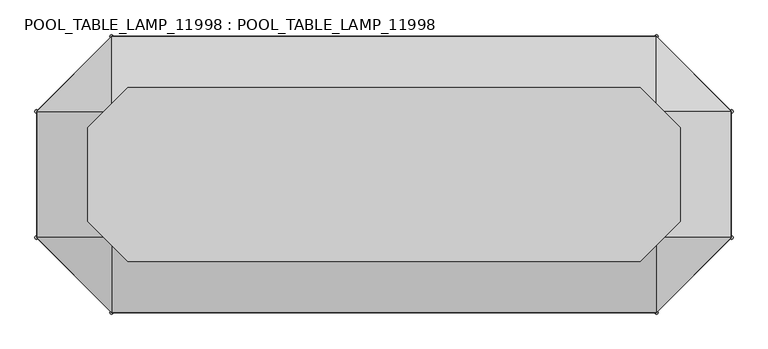
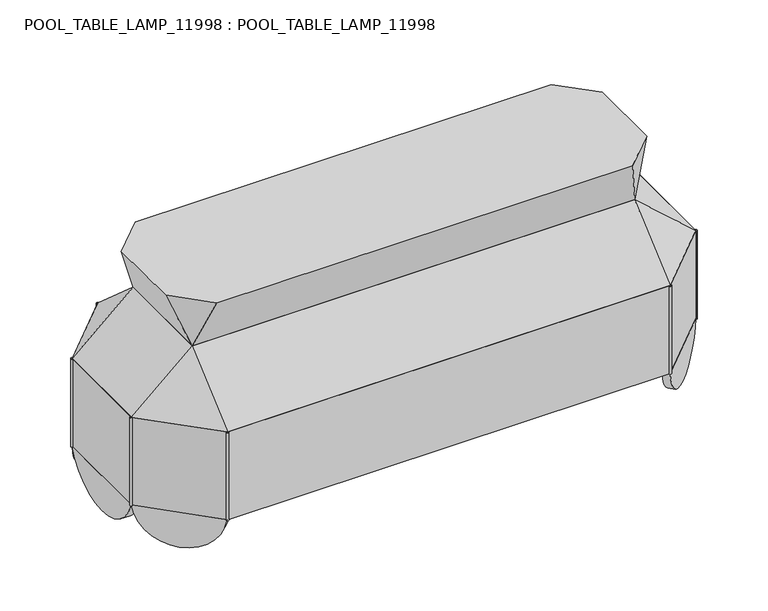
"""IFC4 building model written with IfcOpenShell, lengths in millimetres: proxy geometry, POOL_TABLE_LAMP_11998 : POOL_TABLE_LAMP_11998."""

from ifc_helpers import new_model, si_unit, point, frame, frame_2d, origin, place, context, project, spatial, polyline, circle_curve, trimmed, segment, composite_curve, outline, extrude, faceted_brep, source, transform, mapped, element, save


def pool_table_lamp_11998_pool_table_lamp_11998_d06ee5fc(model_context):
    return source(origin(), model_context, "Body", "SolidModel", [
        extrude(outline(composite_curve([segment(trimmed(circle_curve(frame_2d((246.5034627, 1717.728225)), 130.228225), [point((369.9998934, 1676.4))], [point((123.007032, 1676.4))], False, "CARTESIAN"), True, "CONTINUOUS"), segment(polyline([(123.007032, 1676.4), (369.9998934, 1676.4)]), True, "CONTINUOUS")], self_intersect=False)), frame((-1365.4872204, 0.0, 0.0), z_axis=(1.0, 0.0, 0.0), x_axis=(0.0, 1.0, 0.0)), (0.0, 0.0, 1.0), 24.3292268),
        extrude(outline(composite_curve([segment(polyline([(1676.4, -151.8960871), (1676.4, -685.2960871)]), True, "CONTINUOUS"), segment(trimmed(circle_curve(frame_2d((2032.0, -418.5960871)), 444.5), [point((1676.4, -685.2960871))], [point((1676.4, -151.8960871))], False, "CARTESIAN"), True, "CONTINUOUS")], self_intersect=False)), frame((0.0, 493.0069254, 0.0), z_axis=(0.0, 1.0, 0.0), x_axis=(0.0, 0.0, 1.0)), (0.0, 0.0, 1.0), 24.3292268),
        extrude(outline(composite_curve([segment(trimmed(circle_curve(frame_2d((246.5034627, 1717.728225)), 130.228225), [point((369.9998934, 1676.4))], [point((123.007032, 1676.4))], False, "CARTESIAN"), True, "CONTINUOUS"), segment(polyline([(123.007032, 1676.4), (369.9998934, 1676.4)]), True, "CONTINUOUS")], self_intersect=False)), frame((-29.4341807, 0.0, 0.0), z_axis=(1.0, 0.0, 0.0), x_axis=(0.0, 1.0, 0.0)), (0.0, 0.0, 1.0), 24.3292268),
        extrude(outline(polyline([(-151.8960871, 493.0069254), (-1218.6960871, 493.0069254), (-1218.6960871, 517.3361522), (-151.8960871, 517.3361522), (-151.8960871, 493.0069254)])), frame((0.0, 0.0, 1676.4), z_axis=(0.0, 0.0, 1.0), x_axis=(1.0, 0.0, 0.0)), (0.0, 0.0, 1.0), 224.1601186),
        extrude(outline(polyline([(-1341.1579936, 123.007032), (-1365.4872204, 123.007032), (-1365.4872204, 369.9998934), (-1341.1579936, 369.9998934), (-1341.1579936, 123.007032)])), frame((0.0, 0.0, 1676.4), z_axis=(0.0, 0.0, 1.0), x_axis=(1.0, 0.0, 0.0)), (0.0, 0.0, 1.0), 224.1601186),
        extrude(outline(polyline([(-29.4341807, 123.007032), (-29.4341807, 369.9998934), (-5.1049539, 369.9998934), (-5.1049539, 123.007032), (-29.4341807, 123.007032)])), frame((0.0, 0.0, 1676.4), z_axis=(0.0, 0.0, 1.0), x_axis=(1.0, 0.0, 0.0)), (0.0, 0.0, 1.0), 224.1601186),
        extrude(outline(polyline([(-151.8960871, 0.0), (-151.8960871, -24.3292268), (-1218.6960871, -24.3292268), (-1218.6960871, 0.0), (-151.8960871, 0.0)])), frame((0.0, 0.0, 1676.4), z_axis=(0.0, 0.0, 1.0), x_axis=(1.0, 0.0, 0.0)), (0.0, 0.0, 1.0), 224.1601186),
        extrude(outline(composite_curve([segment(polyline([(-155.0710871, -24.0098052), (-148.7210871, -24.0098052)]), True, "CONTINUOUS"), segment(trimmed(circle_curve(frame_2d((-151.8960871, -24.0098052)), 3.175), [point((-148.7210871, -24.0098052))], [point((-155.0710871, -24.0098052))], False, "CARTESIAN"), True, "CONTINUOUS")], self_intersect=False)), frame((0.0, 0.0, 1676.4), z_axis=(0.0, 0.0, 1.0), x_axis=(1.0, 0.0, 0.0)), (0.0, 0.0, 1.0), 224.1601186),
        extrude(outline(composite_curve([segment(trimmed(circle_curve(frame_2d((-1218.6960871, -24.0098052)), 3.175), [point((-1215.5210871, -24.0098052))], [point((-1221.8710871, -24.0098052))], False, "CARTESIAN"), True, "CONTINUOUS"), segment(polyline([(-1221.8710871, -24.0098052), (-1215.5210871, -24.0098052)]), True, "CONTINUOUS")], self_intersect=False)), frame((0.0, 0.0, 1676.4), z_axis=(0.0, 0.0, 1.0), x_axis=(1.0, 0.0, 0.0)), (0.0, 0.0, 1.0), 224.1601186),
        extrude(outline(composite_curve([segment(polyline([(-1215.5210871, 517.0167306), (-1221.8710871, 517.0167306)]), True, "CONTINUOUS"), segment(trimmed(circle_curve(frame_2d((-1218.6960871, 517.0167306)), 3.175), [point((-1221.8710871, 517.0167306))], [point((-1215.5210871, 517.0167306))], False, "CARTESIAN"), True, "CONTINUOUS")], self_intersect=False)), frame((0.0, 0.0, 1676.4), z_axis=(0.0, 0.0, 1.0), x_axis=(1.0, 0.0, 0.0)), (0.0, 0.0, 1.0), 224.1601186),
        extrude(outline(composite_curve([segment(trimmed(circle_curve(frame_2d((-151.8960871, 517.0167306)), 3.175), [point((-155.0710871, 517.0167306))], [point((-148.7210871, 517.0167306))], False, "CARTESIAN"), True, "CONTINUOUS"), segment(polyline([(-148.7210871, 517.0167306), (-155.0710871, 517.0167306)]), True, "CONTINUOUS")], self_intersect=False)), frame((0.0, 0.0, 1676.4), z_axis=(0.0, 0.0, 1.0), x_axis=(1.0, 0.0, 0.0)), (0.0, 0.0, 1.0), 224.1601186),
        extrude(outline(composite_curve([segment(polyline([(-5.1049539, 119.6063281), (-5.1049539, 125.9563281)]), True, "CONTINUOUS"), segment(trimmed(circle_curve(frame_2d((-5.1049539, 122.7813281)), 3.175), [point((-5.1049539, 125.9563281))], [point((-5.1049539, 119.6063281))], False, "CARTESIAN"), True, "CONTINUOUS")], self_intersect=False)), frame((0.0, 0.0, 1676.4), z_axis=(0.0, 0.0, 1.0), x_axis=(1.0, 0.0, 0.0)), (0.0, 0.0, 1.0), 224.1601186),
        extrude(outline(composite_curve([segment(trimmed(circle_curve(frame_2d((-5.1049539, 370.2255973)), 3.175), [point((-5.1049539, 373.4005973))], [point((-5.1049539, 367.0505973))], False, "CARTESIAN"), True, "CONTINUOUS"), segment(polyline([(-5.1049539, 367.0505973), (-5.1049539, 373.4005973)]), True, "CONTINUOUS")], self_intersect=False)), frame((0.0, 0.0, 1676.4), z_axis=(0.0, 0.0, 1.0), x_axis=(1.0, 0.0, 0.0)), (0.0, 0.0, 1.0), 224.1601186),
        extrude(outline(composite_curve([segment(polyline([(-1365.4872204, 373.4005973), (-1365.4872204, 367.0505973)]), True, "CONTINUOUS"), segment(trimmed(circle_curve(frame_2d((-1365.4872204, 370.2255973)), 3.175), [point((-1365.4872204, 367.0505973))], [point((-1365.4872204, 373.4005973))], False, "CARTESIAN"), True, "CONTINUOUS")], self_intersect=False)), frame((0.0, 0.0, 1676.4), z_axis=(0.0, 0.0, 1.0), x_axis=(1.0, 0.0, 0.0)), (0.0, 0.0, 1.0), 224.1601186),
        extrude(outline(composite_curve([segment(trimmed(circle_curve(frame_2d((-1365.4872204, 122.7813281)), 3.175), [point((-1365.4872204, 119.6063281))], [point((-1365.4872204, 125.9563281))], False, "CARTESIAN"), True, "CONTINUOUS"), segment(polyline([(-1365.4872204, 125.9563281), (-1365.4872204, 119.6063281)]), True, "CONTINUOUS")], self_intersect=False)), frame((0.0, 0.0, 1676.4), z_axis=(0.0, 0.0, 1.0), x_axis=(1.0, 0.0, 0.0)), (0.0, 0.0, 1.0), 224.1601186),
        extrude(outline(composite_curve([segment(polyline([(-207.9132051, 0.0), (0.0, 0.0)]), True, "CONTINUOUS"), segment(trimmed(circle_curve(frame_2d((-103.9566025, 16.3316378)), 105.2316378), [point((0.0, 0.0))], [point((-207.9132051, 0.0))], False, "CARTESIAN"), True, "CONTINUOUS")], self_intersect=False)), frame((-1365.7129243, 123.007032, 1676.4), z_axis=(0.7071067811865518, 0.7071067811865434, 0.0), x_axis=(-0.7071067811865434, 0.7071067811865518, 0.0)), (0.0, 0.0, 1.0), 17.362958),
        extrude(outline(composite_curve([segment(trimmed(circle_curve(frame_2d((0.0, -105.2316378)), 105.2316378), [point((-85.0566304, -167.1918446))], [point((61.9602067, -20.1750074))], False, "CARTESIAN"), True, "CONTINUOUS"), segment(polyline([(61.9602067, -20.1750074), (-85.0566304, -167.1918446)]), True, "CONTINUOUS")], self_intersect=False)), frame((-25.7718496, 102.1144323, 1618.3216331), z_axis=(-0.7071067811865426, 0.7071067811865525, 0.0), x_axis=(0.5000000000000033, 0.4999999999999975, 0.7071067811865469)), (0.0, 0.0, 1.0), 17.362958),
        extrude(outline(composite_curve([segment(polyline([(85.0566304, -167.1918446), (-61.9602067, -20.1750074)]), True, "CONTINUOUS"), segment(trimmed(circle_curve(frame_2d((0.0, -105.2316378)), 105.2316378), [point((-61.9602067, -20.1750074))], [point((85.0566304, -167.1918446))], False, "CARTESIAN"), True, "CONTINUOUS")], self_intersect=False)), frame((-1332.5428593, 378.6150278, 1618.3216331), z_axis=(-0.7071067811865472, 0.7071067811865479, 0.0), x_axis=(0.5000000000000001, 0.5000000000000009, -0.707106781186547)), (0.0, 0.0, 1.0), 17.362958),
        extrude(outline(composite_curve([segment(trimmed(circle_curve(frame_2d((103.9566025, 16.3316378)), 105.2316378), [point((207.9132051, 0.0))], [point((0.0, 0.0))], False, "CARTESIAN"), True, "CONTINUOUS"), segment(polyline([(0.0, 0.0), (207.9132051, 0.0)]), True, "CONTINUOUS")], self_intersect=False)), frame((-17.1567153, 357.7224281, 1676.4), z_axis=(0.7071067811865472, 0.7071067811865479, 0.0), x_axis=(-0.7071067811865479, 0.7071067811865472, 0.0)), (0.0, 0.0, 1.0), 17.362958),
        faceted_brep([(-1218.3766655, 123.007032, 2030.7043208), (-152.2155087, 123.007032, 2030.7043208), (-152.2155087, 369.9998934, 2030.7043208), (-1218.3766655, 369.9998934, 2030.7043208), (-177.484535, 148.453943, 2030.7043208), (-177.6630544, 148.2754236, 2030.7043208), (-1192.9291198, 148.2754236, 2030.7043208), (-1193.1076392, 148.453943, 2030.7043208), (-1193.1076392, 344.5529824, 2030.7043208), (-1192.9291198, 344.7315018, 2030.7043208), (-177.6630544, 344.7315018, 2030.7043208), (-177.484535, 344.5529824, 2030.7043208), (-1365.4872204, 122.7813281, 1900.5601186), (-1365.4872204, 370.2255973, 1900.5601186), (-1218.3766655, 517.3361522, 1900.5601186), (-152.2155087, 517.3361522, 1900.5601186), (-5.1049539, 370.2255973, 1900.5601186), (-5.1049539, 122.7813281, 1900.5601186), (-152.2155087, -24.3292268, 1900.5601186), (-1218.3766655, -24.3292268, 1900.5601186), (-152.4412126, 0.0, 1900.5601186), (-29.4341807, 123.007032, 1900.5601186), (-29.4341807, 369.9998934, 1900.5601186), (-152.4412126, 493.0069254, 1900.5601186), (-1218.1509616, 493.0069254, 1900.5601186), (-1341.1579936, 369.9998934, 1900.5601186), (-1341.1579936, 123.007032, 1900.5601186), (-1218.1509616, 0.0, 1900.5601186), (-177.6155087, 148.407032, 2030.2376392), (-177.6155087, 344.5998934, 2030.2376392), (-1192.9766655, 344.5998934, 2030.2376392), (-1192.9766655, 148.407032, 2030.2376392)], [[[0, 1, 2, 3], [4, 5, 6, 7, 8, 9, 10, 11]], [[12, 13, 14, 15, 16, 17, 18, 19], [20, 21, 22, 23, 24, 25, 26, 27]], [[12, 19, 0]], [[1, 0, 19, 18]], [[18, 17, 1]], [[2, 1, 17, 16]], [[16, 15, 2]], [[3, 2, 15, 14]], [[14, 13, 3]], [[0, 3, 13, 12]], [[4, 28, 5]], [[28, 4, 11, 29]], [[29, 11, 10]], [[29, 10, 9, 30]], [[30, 9, 8]], [[30, 8, 7, 31]], [[31, 7, 6]], [[5, 28, 31, 6]], [[20, 28, 21]], [[21, 28, 29, 22]], [[22, 29, 23]], [[23, 29, 30, 24]], [[24, 30, 25]], [[25, 30, 31, 26]], [[26, 31, 27]], [[28, 20, 27, 31]]]),
        extrude(outline(polyline([(-151.8960871, -24.0098052), (-151.8960871, 0.5451255), (-29.4341807, 123.007032), (-4.87925, 123.007032), (-151.8960871, -24.0098052)])), frame((0.0, 0.0, 1676.4), z_axis=(0.0, 0.0, 1.0), x_axis=(1.0, 0.0, 0.0)), (0.0, 0.0, 1.0), 224.1601186),
        extrude(outline(polyline([(-151.8960871, 517.0167306), (-4.87925, 369.9998934), (-29.4341807, 369.9998934), (-151.8960871, 492.4617999), (-151.8960871, 517.0167306)])), frame((0.0, 0.0, 1676.4), z_axis=(0.0, 0.0, 1.0), x_axis=(1.0, 0.0, 0.0)), (0.0, 0.0, 1.0), 224.1601186),
        extrude(outline(polyline([(-1218.6960871, 517.0167306), (-1218.6960871, 492.4617999), (-1341.1579936, 369.9998934), (-1365.7129243, 369.9998934), (-1218.6960871, 517.0167306)])), frame((0.0, 0.0, 1676.4), z_axis=(0.0, 0.0, 1.0), x_axis=(1.0, 0.0, 0.0)), (0.0, 0.0, 1.0), 224.1601186),
        extrude(outline(polyline([(-1218.6960871, -24.0098052), (-1365.7129243, 123.007032), (-1341.1579936, 123.007032), (-1218.6960871, 0.5451255), (-1218.6960871, -24.0098052)])), frame((0.0, 0.0, 1676.4), z_axis=(0.0, 0.0, 1.0), x_axis=(1.0, 0.0, 0.0)), (0.0, 0.0, 1.0), 224.1601186),
        faceted_brep([(-1186.5878882, 416.8069254, 2157.1484202), (-1264.9579936, 338.43682, 2157.1484202), (-1264.9579936, 154.5701054, 2157.1484202), (-1186.5878882, 76.2, 2157.1484202), (-184.0042861, 76.2, 2157.1484202), (-105.6341807, 154.5701054, 2157.1484202), (-105.6341807, 338.43682, 2157.1484202), (-184.0042861, 416.8069254, 2157.1484202), (-1218.3766655, 369.9998934, 2030.2376392), (-152.2155087, 369.9998934, 2030.2376392), (-152.2155087, 123.007032, 2030.2376392), (-1218.3766655, 123.007032, 2030.2376392)], [[[0, 1, 2, 3, 4, 5, 6, 7]], [[8, 9, 10, 11]], [[1, 0, 8]], [[8, 11, 2, 1]], [[3, 2, 11]], [[11, 10, 4, 3]], [[5, 4, 10]], [[10, 9, 6, 5]], [[7, 6, 9]], [[9, 8, 0, 7]]]),
    ])


if __name__ == "__main__":
    model = new_model("IFC4")
    model_context = context("Model", 3, world=origin())
    ifc_project = project(units=[si_unit("LENGTHUNIT", "METRE", prefix="MILLI")], contexts=[model_context])
    site = spatial("IfcSite", under=ifc_project)
    building = spatial("IfcBuilding", under=site)
    placement = place(None, origin())
    pool_table_lamp_11998_pool_table_lamp_11998_shape = pool_table_lamp_11998_pool_table_lamp_11998_d06ee5fc(model_context)
    element("IfcBuildingElementProxy", 1, Name="POOL_TABLE_LAMP_11998 : POOL_TABLE_LAMP_11998", ObjectType="POOL_TABLE_LAMP_11998 : POOL_TABLE_LAMP_11998", at=placement, inside=building, context=model_context, shape_type="MappedRepresentation", body=[
        mapped(pool_table_lamp_11998_pool_table_lamp_11998_shape, transform((0.0, 0.0, 0.0), x_axis=(1.0, 0.0, 0.0), y_axis=(0.0, 1.0, 0.0), z_axis=(0.0, 0.0, 1.0))),
    ])
    save(model, "model.ifc")

# Revit data of these elements
# Type "POOL_TABLE_LAMP_11998 : POOL_TABLE_LAMP_11998"
#   COBie.Type.CreatedBy = "design@eagle.com"
#   COBie.Type.CreatedOn = "2016-10-27T05:31:12"
#   COBie.Type.Name = "POOL_TABLE_LAMP_11998_POOL_TABLE_LAMP_11998"
#   COBie.Type.Category = "n/a"
#   COBie.Type.Description = "POOL_TABLE_LAMP_11998_POOL_TABLE_LAMP_11998"
#   COBie.Type.Manufacturer = ""
#   COBie.Type.ModelNumber = ""
#   COBie.Type.ReplacementCost = 0
#   Default Elevation = 4' - 0"
#   COBie.Type = yes
# Element 1 (IfcBuildingElementProxy, "POOL_TABLE_LAMP_11998 : POOL_TABLE_LAMP_11998")
#   Materials on its faces: "copper trim 123455", "white glass", "res glass 134"
# Materials
#   "copper trim 123455": class "Metal", colour RGB 187 80 46, transparency 0
#   "white glass": class "Glass", colour RGB 229 229 229, transparency 1
#   "res glass 134": class "Glass", colour RGB 191 25 25, transparency 0.6
